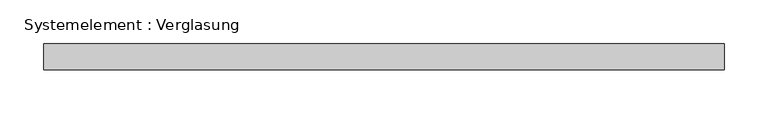
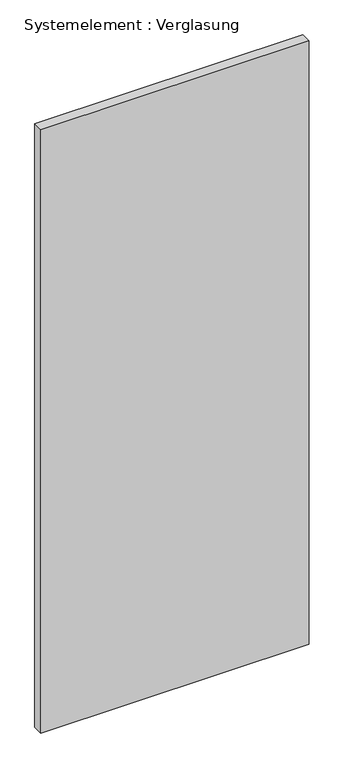
"""IFC4 building model written with IfcOpenShell, lengths in millimetres: plate geometry, Systemelement : Verglasung."""

from ifc_helpers import new_model, si_unit, origin, origin_with_axes, place, context, project, spatial, polyline, outline, extrude, source, transform, mapped, element, save


def systemelement_verglasung_19c2cb46(model_context):
    return source(origin(), model_context, "Body", "SweptSolid", [
        extrude(outline(polyline([(390.3580711, -15.0), (-390.3580711, -15.0), (-390.3580711, 15.0), (390.3580711, 15.0), (390.3580711, -15.0)])), origin_with_axes(), (0.0, 0.0, 1.0), 1856.6788019),
    ])


if __name__ == "__main__":
    model = new_model("IFC4")
    model_context = context("Model", 3, world=origin())
    ifc_project = project(units=[si_unit("LENGTHUNIT", "METRE", prefix="MILLI")], contexts=[model_context])
    site = spatial("IfcSite", under=ifc_project)
    building = spatial("IfcBuilding", under=site)
    placement = place(None, origin())
    systemelement_verglasung_shape = systemelement_verglasung_19c2cb46(model_context)
    element("IfcPlate", 1, ObjectType="Systemelement : Verglasung", at=placement, inside=building, context=model_context, shape_type="MappedRepresentation", body=[
        mapped(systemelement_verglasung_shape, transform((0.0, 0.0, 0.0), x_axis=(1.0, 0.0, 0.0), y_axis=(0.0, 1.0, 0.0), z_axis=(0.0, 0.0, 1.0))),
    ])
    save(model, "model.ifc")

# Revit data of these elements
# Type "Systemelement : Verglasung"
#   Construction Type Id = "GSP4R"
#   Analytic Construction = "1/8 Zoll Pilkington-Verglasung einfach"
#   Visual Light Transmittance = 0.9
#   Solar Heat Gain Coefficient = 0.86
#   Heat Transfer Coefficient (U) = 6.7069 W/(m²·K)
# Element 1 (IfcPlate, "Systemelement : Verglasung")
#   Materials on its faces: "Glas"
# Materials
#   "Glas": class "Glas", colour RGB 0 0 255, transparency 0.75, Comments = "Render-Darstellung nicht aktualisiert ", Cost = 0
